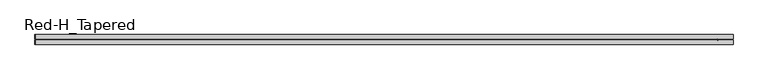
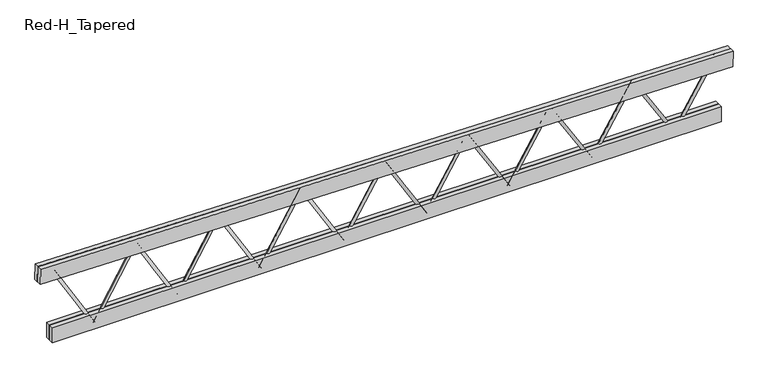
"""IFC4 building model written with IfcOpenShell, lengths in millimetres: beam geometry, Construction_Frames_RedBuilt_Openweb_Red-H_Tapered : Red-H_Tapered."""

import ifcopenshell
import ifcopenshell.guid

model = None  # the IFC model being written
_history = None  # IfcOwnerHistory: only IFC2X3 demands one
_inside = {}  # id of a spatial element -> (the spatial element, [elements in it])
_under = {}  # id of a project, library or spatial element -> (it, [spatial elements below it])
_declared = {}  # id of a project -> (the project, [libraries it declares])
_typed = {}  # id of a type object -> (the type object, [elements of that type])
_made_of = {}  # id of a material, layer set ... -> (it, [elements and type objects made of it])


def new_model(schema):
    """Start an empty IFC model of exactly this schema.

    Asked for "IFC4X3", IfcOpenShell would pick the latest addendum, in which some entities
    have other attributes; the version numbers below select the first issue.
    IFC2X3 requires an IfcOwnerHistory on every rooted entity: one is made here for all.
    """
    global model, _history
    if schema == "IFC4X3":
        model = ifcopenshell.file(schema_version=(4, 3, 0, 0))
    else:
        model = ifcopenshell.file(schema=schema)
    _inside.clear()
    _under.clear()
    _declared.clear()
    _typed.clear()
    _made_of.clear()
    _history = None
    if model.schema == "IFC2X3":
        org = make("IfcOrganization", Name="unknown")
        user = make(
            "IfcPersonAndOrganization",
            ThePerson=make("IfcPerson", FamilyName="unknown"),
            TheOrganization=org,
        )
        app = make(
            "IfcApplication",
            ApplicationDeveloper=org,
            Version="unknown",
            ApplicationFullName="unknown",
            ApplicationIdentifier="unknown",
        )
        _history = make(
            "IfcOwnerHistory",
            OwningUser=user,
            OwningApplication=app,
            ChangeAction="ADDED",
            CreationDate=0,
        )
    return model


def make(cls, **values):
    """One entity of the class cls with the attributes given. An attribute that is None is left unset."""
    return model.create_entity(
        cls, **{name: value for name, value in values.items() if value is not None}
    )


def rooted(cls, **values):
    """An entity with a GlobalId (a new one), such as an element, a storey or a relation."""
    return make(cls, GlobalId=ifcopenshell.guid.new(), OwnerHistory=_history, **values)


def si_unit(unit_type, name, prefix=None):
    """IfcSIUnit, for example si_unit("LENGTHUNIT", "METRE", prefix="MILLI")."""
    return make("IfcSIUnit", UnitType=unit_type, Prefix=prefix, Name=name)


def assignment(units):
    """IfcUnitAssignment: the units of a project."""
    return None if units is None else make("IfcUnitAssignment", Units=units)


def point(xyz):
    """IfcCartesianPoint."""
    return None if xyz is None else make("IfcCartesianPoint", Coordinates=xyz)


def direction(xyz):
    """IfcDirection."""
    return None if xyz is None else make("IfcDirection", DirectionRatios=xyz)


def frame(location, z_axis=None, x_axis=None):
    """IfcAxis2Placement3D, a coordinate frame: its origin and axes. An axis left out is left unset."""
    return make(
        "IfcAxis2Placement3D",
        Location=point(location),
        Axis=direction(z_axis),
        RefDirection=direction(x_axis),
    )


def frame_2d(location, x_axis=None):
    """IfcAxis2Placement2D, a coordinate frame in the plane: its origin and x axis."""
    return make(
        "IfcAxis2Placement2D", Location=point(location), RefDirection=direction(x_axis)
    )


def origin():
    """The frame at (0, 0, 0) with its axes left unset."""
    return frame((0.0, 0.0, 0.0))


def origin_2d():
    """The frame at (0, 0) in the plane with its x axis left unset."""
    return frame_2d((0.0, 0.0))


def place(relative_to, where):
    """IfcLocalPlacement: puts the frame where relative to a parent placement (None: the world)."""
    return make(
        "IfcLocalPlacement", PlacementRelTo=relative_to, RelativePlacement=where
    )


def context(
    kind, dimensions, precision=None, world=None, true_north=None, identifier=None
):
    """IfcGeometricRepresentationContext, for example the 3D "Model" context."""
    return make(
        "IfcGeometricRepresentationContext",
        ContextIdentifier=identifier,
        ContextType=kind,
        CoordinateSpaceDimension=dimensions,
        Precision=precision,
        WorldCoordinateSystem=world,
        TrueNorth=true_north,
    )


def project(units=None, contexts=None):
    """IfcProject with its units and contexts."""
    return rooted(
        "IfcProject",
        Name="project",
        RepresentationContexts=contexts,
        UnitsInContext=assignment(units),
    )


def spatial(cls, under=None, at=None, **own):
    """A site, building, storey or space (cls), placed at a placement, below another one or the project."""
    s = rooted(cls, ObjectPlacement=at, **own)
    if under is not None:
        _under.setdefault(under.id(), (under, []))[1].append(s)
    return s


def polyline(points):
    """IfcPolyline through the points."""
    return make("IfcPolyline", Points=[point(p) for p in points])


def circle_curve(where, radius):
    """IfcCircle in the frame where."""
    return make("IfcCircle", Position=where, Radius=radius)


def trimmed(basis, trim1, trim2, sense, master):
    """IfcTrimmedCurve: the piece of a basis curve between two trims."""
    return make(
        "IfcTrimmedCurve",
        BasisCurve=basis,
        Trim1=trim1,
        Trim2=trim2,
        SenseAgreement=sense,
        MasterRepresentation=master,
    )


def segment(curve, same_sense, transition):
    """IfcCompositeCurveSegment."""
    return make(
        "IfcCompositeCurveSegment",
        Transition=transition,
        SameSense=same_sense,
        ParentCurve=curve,
    )


def composite_curve(segments, self_intersect=None):
    """IfcCompositeCurve: segments joined end to end."""
    return make("IfcCompositeCurve", Segments=segments, SelfIntersect=self_intersect)


def outline(outer, holes=None, kind="AREA"):
    """IfcArbitraryClosedProfileDef: a profile drawn as a closed curve; with holes, ...WithVoids."""
    if holes is None:
        return make("IfcArbitraryClosedProfileDef", ProfileType=kind, OuterCurve=outer)
    return make(
        "IfcArbitraryProfileDefWithVoids",
        ProfileType=kind,
        OuterCurve=outer,
        InnerCurves=holes,
    )


def extrude(swept, where, along, depth):
    """IfcExtrudedAreaSolid: the profile swept, set in the frame where, extruded along a direction by depth."""
    return make(
        "IfcExtrudedAreaSolid",
        SweptArea=swept,
        Position=where,
        ExtrudedDirection=direction(along),
        Depth=depth,
    )


def shape(context_of_items, identifier, shape_type, items):
    """IfcShapeRepresentation: the items that make up one representation, for example the "Body"."""
    return make(
        "IfcShapeRepresentation",
        ContextOfItems=context_of_items,
        RepresentationIdentifier=identifier,
        RepresentationType=shape_type,
        Items=items,
    )


def source(mapping_origin, context_of_items, identifier, shape_type, items):
    """IfcRepresentationMap: a shape defined once, which mapped items show again and again."""
    return make(
        "IfcRepresentationMap",
        MappingOrigin=mapping_origin,
        MappedRepresentation=shape(context_of_items, identifier, shape_type, items),
    )


def transform(
    local_origin,
    x_axis=None,
    y_axis=None,
    z_axis=None,
    scale=None,
    scale2=None,
    scale3=None,
    uniform=True,
):
    """IfcCartesianTransformationOperator3D, or its non-uniform kind. x_axis, y_axis, z_axis: its Axis1, 2, 3."""
    if uniform:
        return make(
            "IfcCartesianTransformationOperator3D",
            Axis1=direction(x_axis),
            Axis2=direction(y_axis),
            LocalOrigin=point(local_origin),
            Scale=scale,
            Axis3=direction(z_axis),
        )
    return make(
        "IfcCartesianTransformationOperator3DnonUniform",
        Axis1=direction(x_axis),
        Axis2=direction(y_axis),
        LocalOrigin=point(local_origin),
        Scale=scale,
        Axis3=direction(z_axis),
        Scale2=scale2,
        Scale3=scale3,
    )


def mapped(mapping_source, mapping_target):
    """IfcMappedItem: shows the shape of a source again, moved by a transform."""
    return make(
        "IfcMappedItem", MappingSource=mapping_source, MappingTarget=mapping_target
    )


def made_of(thing, what):
    """Note that an element or type object is made of a material, layer set ...; save() writes the relation."""
    if what is not None:
        _made_of.setdefault(what.id(), (what, []))[1].append(thing)
    return thing


def element(
    cls,
    number,
    at=None,
    inside=None,
    cuts=None,
    type_object=None,
    material=None,
    context=None,
    identifier="Body",
    shape_type=None,
    held_by="IfcProductDefinitionShape",
    body=None,
    shapes=None,
    **own,
):
    """One element of the class cls, such as IfcWall. Its Tag is "e" and its number.

    at: its placement. inside: the storey or other place that contains it. cuts: it is an
    opening in that element (IfcRelVoidsElement). A single representation is given by context,
    identifier, shape_type and body (its items); several are given by shapes. held_by: the class
    of the entity that holds the representations. save() writes the other relations.
    """
    e = rooted(cls, Tag="e%d" % number, ObjectPlacement=at, **own)
    if body is not None:
        shapes = [shape(context, identifier, shape_type, body)]
    if shapes is not None:
        e.Representation = make(held_by, Representations=shapes)
    if inside is not None:
        _inside.setdefault(inside.id(), (inside, []))[1].append(e)
    if cuts is not None:
        rooted(
            "IfcRelVoidsElement", RelatingBuildingElement=cuts, RelatedOpeningElement=e
        )
    if type_object is not None:
        _typed.setdefault(type_object.id(), (type_object, []))[1].append(e)
    return made_of(e, material)


def aggregate(whole, parts):
    """IfcRelAggregates: a whole, such as a stair, and the parts it consists of."""
    return rooted("IfcRelAggregates", RelatingObject=whole, RelatedObjects=parts)


def save(model, path):
    """Write the relations noted so far, then the file.

    IfcRelAggregates (storeys below a building ...), IfcRelContainedInSpatialStructure (elements
    in a storey), IfcRelDefinesByType, IfcRelAssociatesMaterial and IfcRelDeclares: one each for
    every whole, place, type object, material and project.
    """
    for whole, parts in _under.values():
        aggregate(whole, parts)
    for where, things in _inside.values():
        rooted(
            "IfcRelContainedInSpatialStructure",
            RelatedElements=things,
            RelatingStructure=where,
        )
    for kind, things in _typed.values():
        rooted("IfcRelDefinesByType", RelatedObjects=things, RelatingType=kind)
    for what, things in _made_of.values():
        rooted("IfcRelAssociatesMaterial", RelatedObjects=things, RelatingMaterial=what)
    for by, libraries in _declared.values():
        rooted("IfcRelDeclares", RelatingContext=by, RelatedDefinitions=libraries)
    model.write(path)


def red_h_tapered_5ce7bd37(model_context):
    return source(origin(), model_context, "Body", "SweptSolid", [
        extrude(outline(composite_curve([segment(trimmed(circle_curve(origin_2d(), 12.7), [point((0.0, 12.7))], [point((0.0, -12.7))], False, "CARTESIAN"), True, "CONTINUOUS"), segment(trimmed(circle_curve(origin_2d(), 12.7), [point((0.0, -12.7))], [point((0.0, 12.7))], False, "CARTESIAN"), True, "CONTINUOUS")], self_intersect=False)), frame((2516.6154336, 0.0, -367.0101562), z_axis=(0.5241067286958753, 0.0, 0.8516525916920046), x_axis=(0.0, -1.0, 0.0)), (0.0, 0.0, 1.0), 685.9604558),
        extrude(outline(composite_curve([segment(trimmed(circle_curve(origin_2d(), 12.7), [point((0.0, -12.7))], [point((0.0, 12.6999999))], False, "CARTESIAN"), True, "CONTINUOUS"), segment(trimmed(circle_curve(origin_2d(), 12.7), [point((0.0, 12.6999999))], [point((0.0, -12.7))], False, "CARTESIAN"), True, "CONTINUOUS")], self_intersect=False)), frame((2516.6154336, 0.0, -367.0101562), z_axis=(-0.5215353438102012, 0.0, 0.853229679017775), x_axis=(0.0, -1.0, 0.0)), (0.0, 0.0, 1.0), 689.3425245),
        extrude(outline(composite_curve([segment(trimmed(circle_curve(origin_2d(), 12.7), [point((0.0, 12.7))], [point((0.0, -12.6999999))], False, "CARTESIAN"), True, "CONTINUOUS"), segment(trimmed(circle_curve(origin_2d(), 12.7), [point((0.0, -12.6999999))], [point((0.0, 12.7))], False, "CARTESIAN"), True, "CONTINUOUS")], self_intersect=False)), frame((1797.5824526, 0.0, -367.0101562), z_axis=(0.5215353438102003, 0.0, 0.8532296790177755), x_axis=(0.0, -1.0, 0.0)), (0.0, 0.0, 1.0), 689.3425245),
        extrude(outline(composite_curve([segment(trimmed(circle_curve(origin_2d(), 12.7), [point((0.0, -12.7))], [point((0.0, 12.7))], False, "CARTESIAN"), True, "CONTINUOUS"), segment(trimmed(circle_curve(origin_2d(), 12.7), [point((0.0, 12.7))], [point((0.0, -12.7))], False, "CARTESIAN"), True, "CONTINUOUS")], self_intersect=False)), frame((1797.5824526, 0.0, -367.0101562), z_axis=(-0.5189844139237941, 0.0, 0.8547837025260694), x_axis=(0.0, -1.0, 0.0)), (0.0, 0.0, 1.0), 692.7308044),
        extrude(outline(composite_curve([segment(trimmed(circle_curve(origin_2d(), 12.7), [point((0.0, 12.7000001))], [point((0.0, -12.7))], False, "CARTESIAN"), True, "CONTINUOUS"), segment(trimmed(circle_curve(origin_2d(), 12.7), [point((0.0, -12.7))], [point((0.0, 12.7000001))], False, "CARTESIAN"), True, "CONTINUOUS")], self_intersect=False)), frame((1078.5494715, 0.0, -367.0101562), z_axis=(0.518984413923793, 0.0, 0.8547837025260702), x_axis=(0.0, -1.0, 0.0)), (0.0, 0.0, 1.0), 692.7308044),
        extrude(outline(composite_curve([segment(trimmed(circle_curve(origin_2d(), 12.7), [point((0.0, -12.7))], [point((0.0, 12.7))], False, "CARTESIAN"), True, "CONTINUOUS"), segment(trimmed(circle_curve(origin_2d(), 12.7), [point((0.0, 12.7))], [point((0.0, -12.7))], False, "CARTESIAN"), True, "CONTINUOUS")], self_intersect=False)), frame((1078.5494715, 0.0, -367.0101562), z_axis=(-0.5164537759218651, 0.0, 0.856315068964717), x_axis=(0.0, -1.0, 0.0)), (0.0, 0.0, 1.0), 696.1252048),
        extrude(outline(composite_curve([segment(trimmed(circle_curve(origin_2d(), 12.7), [point((0.0, 12.7))], [point((0.0, -12.7))], False, "CARTESIAN"), True, "CONTINUOUS"), segment(trimmed(circle_curve(origin_2d(), 12.7), [point((0.0, -12.7))], [point((0.0, 12.7))], False, "CARTESIAN"), True, "CONTINUOUS")], self_intersect=False)), frame((359.5164905, 0.0, -367.0101562), z_axis=(0.5164537759218657, 0.0, 0.8563150689647167), x_axis=(0.0, -1.0, 0.0)), (0.0, 0.0, 1.0), 696.1252048),
        extrude(outline(composite_curve([segment(trimmed(circle_curve(origin_2d(), 12.7), [point((0.0, -12.7))], [point((0.0, 12.7))], False, "CARTESIAN"), True, "CONTINUOUS"), segment(trimmed(circle_curve(origin_2d(), 12.7), [point((0.0, 12.7))], [point((0.0, -12.7))], False, "CARTESIAN"), True, "CONTINUOUS")], self_intersect=False)), frame((359.5164905, 0.0, -367.0101562), z_axis=(-0.5139432662956527, 0.0, 0.8578241772236056), x_axis=(0.0, -1.0, 0.0)), (0.0, 0.0, 1.0), 699.5256366),
        extrude(outline(composite_curve([segment(trimmed(circle_curve(origin_2d(), 12.7), [point((0.0, -12.7))], [point((0.0, 12.7))], False, "CARTESIAN"), True, "CONTINUOUS"), segment(trimmed(circle_curve(origin_2d(), 12.7), [point((0.0, 12.7))], [point((0.0, -12.7))], False, "CARTESIAN"), True, "CONTINUOUS")], self_intersect=False)), frame((-359.5164905, 0.0, -367.0101562), z_axis=(0.5139432662956213, 0.0, 0.8578241772236244), x_axis=(0.0, -1.0, 0.0)), (0.0, 0.0, 1.0), 699.5256366),
        extrude(outline(composite_curve([segment(trimmed(circle_curve(origin_2d(), 12.7), [point((0.0, 12.7))], [point((0.0, -12.7))], False, "CARTESIAN"), True, "CONTINUOUS"), segment(trimmed(circle_curve(origin_2d(), 12.7), [point((0.0, -12.7))], [point((0.0, 12.7))], False, "CARTESIAN"), True, "CONTINUOUS")], self_intersect=False)), frame((-359.5164905, 0.0, -367.0101562), z_axis=(-0.511452721242837, 0.0, 0.8593114184818545), x_axis=(0.0, -1.0, 0.0)), (0.0, 0.0, 1.0), 702.9320123),
        extrude(outline(composite_curve([segment(trimmed(circle_curve(origin_2d(), 12.7), [point((0.0, -12.7))], [point((0.0, 12.7))], False, "CARTESIAN"), True, "CONTINUOUS"), segment(trimmed(circle_curve(origin_2d(), 12.7), [point((0.0, 12.7))], [point((0.0, -12.7))], False, "CARTESIAN"), True, "CONTINUOUS")], self_intersect=False)), frame((-1078.5494715, 0.0, -367.0101562), z_axis=(0.5114527212428354, 0.0, 0.8593114184818554), x_axis=(0.0, -1.0, 0.0)), (0.0, 0.0, 1.0), 702.9320123),
        extrude(outline(composite_curve([segment(trimmed(circle_curve(origin_2d(), 12.7), [point((0.0, 12.7))], [point((0.0, -12.7000001))], False, "CARTESIAN"), True, "CONTINUOUS"), segment(trimmed(circle_curve(origin_2d(), 12.7), [point((0.0, -12.7000001))], [point((0.0, 12.7))], False, "CARTESIAN"), True, "CONTINUOUS")], self_intersect=False)), frame((-1078.5494715, 0.0, -367.0101562), z_axis=(-0.5089819767631879, 0.0, 0.8607771763529966), x_axis=(0.0, -1.0, 0.0)), (0.0, 0.0, 1.0), 706.3442458),
        extrude(outline(composite_curve([segment(trimmed(circle_curve(origin_2d(), 12.7), [point((0.0, -12.7))], [point((0.0, 12.7000001))], False, "CARTESIAN"), True, "CONTINUOUS"), segment(trimmed(circle_curve(origin_2d(), 12.7), [point((0.0, 12.7000001))], [point((0.0, -12.7))], False, "CARTESIAN"), True, "CONTINUOUS")], self_intersect=False)), frame((-1797.5824526, 0.0, -367.0101562), z_axis=(0.508981976763201, 0.0, 0.8607771763529889), x_axis=(0.0, -1.0, 0.0)), (0.0, 0.0, 1.0), 706.3442458),
        extrude(outline(composite_curve([segment(trimmed(circle_curve(origin_2d(), 12.7), [point((0.0, 12.7))], [point((0.0, -12.7))], False, "CARTESIAN"), True, "CONTINUOUS"), segment(trimmed(circle_curve(origin_2d(), 12.7), [point((0.0, -12.7))], [point((0.0, 12.7))], False, "CARTESIAN"), True, "CONTINUOUS")], self_intersect=False)), frame((-1797.5824526, 0.0, -367.0101562), z_axis=(-0.5065308687490784, 0.0, 0.8622218270284648), x_axis=(0.0, -1.0, 0.0)), (0.0, 0.0, 1.0), 709.7622528),
        extrude(outline(composite_curve([segment(trimmed(circle_curve(origin_2d(), 12.7), [point((0.0, -12.7))], [point((0.0, 12.7))], False, "CARTESIAN"), True, "CONTINUOUS"), segment(trimmed(circle_curve(origin_2d(), 12.7), [point((0.0, 12.7))], [point((0.0, -12.7))], False, "CARTESIAN"), True, "CONTINUOUS")], self_intersect=False)), frame((-2516.6154336, 0.0, -367.0101562), z_axis=(0.5065308687490667, 0.0, 0.8622218270284718), x_axis=(0.0, -1.0, 0.0)), (0.0, 0.0, 1.0), 709.7622528),
        extrude(outline(composite_curve([segment(trimmed(circle_curve(origin_2d(), 12.7), [point((0.0, 12.7))], [point((0.0, -12.7))], False, "CARTESIAN"), True, "CONTINUOUS"), segment(trimmed(circle_curve(origin_2d(), 12.7), [point((0.0, -12.7))], [point((0.0, 12.7))], False, "CARTESIAN"), True, "CONTINUOUS")], self_intersect=False)), frame((-2516.6154336, 0.0, -367.0101562), z_axis=(-0.5040992330715739, 0.0, 0.8636457394190346), x_axis=(0.0, -1.0, 0.0)), (0.0, 0.0, 1.0), 713.1859502),
        extrude(outline(polyline([(-2901.5319241, -41.275), (-2901.5319241, -3.175), (2901.5319241, -3.175), (2901.5319241, -41.275), (-2901.5319241, -41.275)])), frame((0.0, 0.0, -386.0601562), z_axis=(0.0, 0.0, 1.0), x_axis=(1.0, 0.0, 0.0)), (0.0, 0.0, 1.0), 139.7),
        extrude(outline(polyline([(-2901.5319241, 3.175), (-2901.5319241, 41.275), (2901.5319241, 41.275), (2901.5319241, 3.175), (-2901.5319241, 3.175)])), frame((0.0, 0.0, -386.0601562), z_axis=(0.0, 0.0, 1.0), x_axis=(1.0, 0.0, 0.0)), (0.0, 0.0, 1.0), 139.7),
        extrude(outline(polyline([(0.0, -38.1), (0.0, 0.0), (6007.123103, 0.0), (6007.123103, -38.1), (0.0, -38.1)])), frame((-3005.4947057, -3.175, 185.4598263), z_axis=(0.016913254191312635, 0.0, 0.9998569606862074), x_axis=(0.9998569606862074, 0.0, -0.016913254191312635)), (0.0, 0.0, 1.0), 139.7),
        extrude(outline(polyline([(0.0, -38.1), (0.0, 0.0), (6007.123103, 0.0), (6007.123103, -38.1), (0.0, -38.1)])), frame((-3005.4947057, 41.275, 185.4598263), z_axis=(0.016913254191312635, 0.0, 0.9998569606862074), x_axis=(0.9998569606862074, 0.0, -0.016913254191312635)), (0.0, 0.0, 1.0), 139.7),
    ])


if __name__ == "__main__":
    model = new_model("IFC4")
    model_context = context("Model", 3, world=origin())
    ifc_project = project(units=[si_unit("LENGTHUNIT", "METRE", prefix="MILLI")], contexts=[model_context])
    site = spatial("IfcSite", under=ifc_project)
    building = spatial("IfcBuilding", under=site)
    placement = place(None, origin())
    red_h_tapered_shape = red_h_tapered_5ce7bd37(model_context)
    element("IfcBeam", 1, ObjectType="Construction_Frames_RedBuilt_Openweb_Red-H_Tapered : Red-H_Tapered", at=placement, inside=building, context=model_context, shape_type="MappedRepresentation", body=[
        mapped(red_h_tapered_shape, transform((0.0, 0.0, 0.0), x_axis=(1.0, 0.0, 0.0), y_axis=(0.0, 1.0, 0.0), z_axis=(0.0, 0.0, 1.0))),
    ])
    save(model, "model.ifc")

# Revit data of these elements
# Type "Construction_Frames_RedBuilt_Openweb_Red-H_Tapered : Red-H_Tapered"
#   Youtube clip = ""
#   Weight Net (Kg) = "0"
#   Webs = "Up to 2\" diameter tubular steel"
#   Uniformat II Description = ""
#   Uniformat II Code = ""
#   Uniclass 2015 Name = "Softwood trusses"
#   Uniclass 2015 Code = "Pr_20_85_90_81"
#   Uniclass 2.0 Description = "Structural Framing Systems"
#   Uniclass 2.0 Code = "SS-15-10-75"
#   Uniclass 1.4 Description = "Trusses"
#   Uniclass 1.4 Code = "L3523"
#   UNSPSC Code = "30103606"
#   Technical description = "http://www.redbuilt.com/reference/literature-and-other-resources"
#   Region South America = "None"
#   Region Oceania = "None"
#   Region North America = "US"
#   Region Middle East = "None"
#   Region Europe = "None"
#   Region Asia = "None"
#   Region Antarctica = "None"
#   Region Africa = "None"
#   QR code = "http://bimobject.com/redbuilt/product/redbuilt-0003"
#   Product url = "http://www.redbuilt.com/products/default.aspx?id=2"
#   Product group = "Wood Trusses"
#   Product family = "Construction"
#   Product data url = "https://bimobject.com/redbuilt/product/redbuilt-0003"
#   Product certification = ""
#   Product SKU = "redbuilt-0003"
#   Product Page URL = "http://www.redbuilt.com/commercial-systems/red-m-red-h-open-web-trusses"
#   Product Guid = "2c5793f2-6ffb-4665-b825-cf90c048e711"
#   Product Documentation Link = "http://www.redbuilt.com/documents/OW_Guide_2017_07_LowRes_wLinks.pdf"
#   OmniClass Description = "Wood Trusses"
#   OmniClass Code = "23-13 35 19 13 17"
#   NBS Reference Description = ""
#   NBS Reference Code = ""
#   Material secondary = "Steel"
#   Material main = "CHARRED WOOD"
#   Masterformat 2014 Description = "Metal-Web Wood Joists"
#   Masterformat 2014 Code = "06 17 36"
#   Manufacturer name = "RedBuilt"
#   Manufacturer country = "United States"
#   Installation instructions = "http://www.redbuilt.com/documents/Installation_Sheets_Open-Web.pdf"
#   IFC Classification = ""
#   EAN code = ""
#   Design country = "United States"
#   Product Information = "http://redbuilt.com/products/default.aspx?id=2"
#   Model = "Red-H-Tapered"
#   Manufacturer URL = "http://redbuilt.com/"
#   Manufacturer = "RedBuilt™"
#   Description = "Open Web Truss"
#   Date of publishing = "8/17/2010"
#   Contact us = "http://redbuilt.com/contact/"
#   Chords = "Double 1½\" x 5½\" MSR lumber"
#   COBIe Type Category = ""
#   Brand url = "http://www.redbuilt.com"
#   BIMobject main category code = "construction"
#   BIMobject main category = "Construction"
#   BIMobject category code = "construction-frames-trusses"
#   BIMobject category = "Frames & Trusses"
#   Web Radius = 0' - 0 1/2"
#   Web Layout Offset Start [instance default] = 0' - 5"
#   Web Layout Offset End [instance default] = 0' - 5"
#   Web Diameter = 0' - 1"
#   TotalLength [instance default] = 20' - 0"
#   Span Minimum = 4' - 0"
#   Span Maximum = 70' - 0"
#   Span Limit [instance default] = 20' - 0"
#   Nominal width = 0' - 0"
#   Nominal height = 0' - 0"
#   Inner Depth Top [instance default] = 0' - 2.76372"
#   Depth Start [instance default] = 6' - 0"
#   Top Chord Length [instance default] = 20' - 1.19701"
#   TC Extension Start Aux [instance default] = 0' - 0"
#   TC Extension End Aux [instance default] = 0' - 0"
#   T-B Chord Length Difference L [instance default] = 0' - 4"
#   T-B Chord Length Difference [instance default] = 0' - 4"
#   Height 2 [instance default] = 6' - 0"
#   Depth Minimum at Wall = 2' - 0"
#   Depth Maximum at Wall = 6' - 0"
#   Depth Lower End [instance default] = 2' - 0"
#   Depth Higher End [instance default] = 6' - 0"
#   Depth End [instance default] = 2' - 0"
#   Depth 2 [instance default] = 2' - 0"
#   Chord Width = 0' - 3 1/4"
#   Chord Thickness = 0' - 1 1/2"
#   Chord Depth = 0' - 5 1/2"
#   Offset Start [instance default] = 0' - 0"
#   TC Extension Start [instance default] = 0' - 0"
#   End Panel = 0' - 5"
#   Offset End [instance default] = 0' - 0"
#   TC Extension End [instance default] = 0' - 0"
#   Length [instance default] = 20' - 0"
#   Angle [instance default] = 5.71059°
#   Span Limit Warning [instance default] = no
#   Edition number = 1
#   Top Bearing Start [instance default] = yes
#   Top Bearing End [instance default] = yes
#   Bottom Bearing Start [instance default] = no
#   Bottom Bearing End [instance default] = no
#   8 Panels [instance default] = yes
#   16 Panels [instance default] = no
#   12 Panels [instance default] = no
#   Web Material = RedBuilt-Steel, Galvanized
#   Clip Material = RedBuilt-Steel, Galvanized
#   Chords Material = WOOD-OAKFIRE
#   URL = ""
#   Assembly Code = ""
# Element 1 (IfcBeam, "Construction_Frames_RedBuilt_Openweb_Red-H_Tapered : Red-H_Tapered")
#   TotalLength = 19' - 8.46708"
#   Span Limit = 19' - 8.46708"
#   Inner Depth Top = 0' - 2.75039"
#   Depth Start = 5' - 0"
#   Top Chord Length = 19' - 8.50091"
#   Height 2 = 5' - 0"
#   Depth Higher End = 5' - 0"
#   Depth 2 = 0' - 4"
#   Angle = 0.969104°
#   Materials on its faces: "RedBuilt-Steel, Galvanized", "WOOD-OAKFIRE"
# Materials
#   "RedBuilt-Steel, Galvanized": class "Metal", colour RGB 164 172 176, transparency 0, Manufacturer = "RedBuilt. LLC", Comments = "Openweb Metal Web", URL = "http://www.redbuilt.com/", Description = "Galvanized steel", Cost = 0
#   "WOOD-OAKFIRE": class "Wood", colour RGB 198 202 183, transparency 0, Description = "Generic wood", Cost = 0
